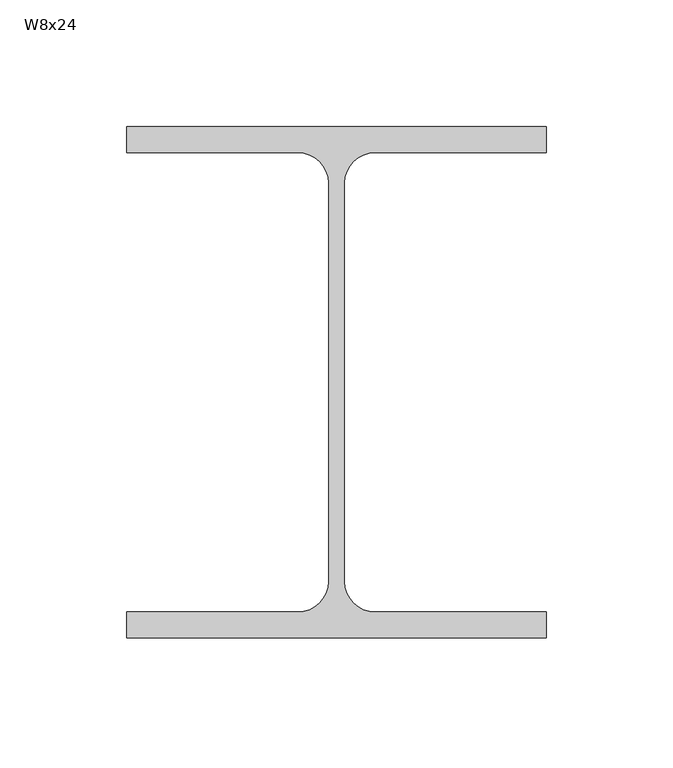
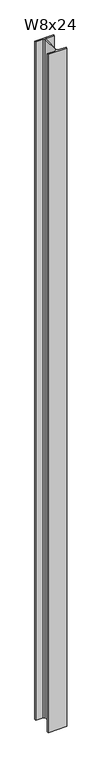
"""IFC4 building model written with IfcOpenShell, lengths in millimetres: column geometry, RME WF - Column : W8x24."""

from ifc_helpers import new_model, si_unit, point, frame, frame_2d, origin, place, context, project, spatial, polyline, circle_curve, trimmed, segment, composite_curve, outline, extrude, source, transform, mapped, element, save


def w8x24_ef2073df(model_context):
    return source(origin(), model_context, "Body", "SweptSolid", [
        extrude(outline(composite_curve([segment(polyline([(82.55, 100.711), (82.55, 90.551), (15.1765, 90.551)]), True, "CONTINUOUS"), segment(trimmed(circle_curve(frame_2d((15.1765, 78.486)), 12.065), [point((15.1765, 90.551))], [point((3.1115, 78.486))], True, "CARTESIAN"), True, "CONTINUOUS"), segment(polyline([(3.1115, 78.486), (3.1115, -78.486)]), True, "CONTINUOUS"), segment(trimmed(circle_curve(frame_2d((15.1765, -78.486)), 12.065), [point((3.1115, -78.486))], [point((15.1765, -90.551))], True, "CARTESIAN"), True, "CONTINUOUS"), segment(polyline([(15.1765, -90.551), (82.55, -90.551), (82.55, -100.711), (-82.55, -100.711), (-82.55, -90.551), (-15.1765, -90.551)]), True, "CONTINUOUS"), segment(trimmed(circle_curve(frame_2d((-15.1765, -78.486)), 12.065), [point((-15.1765, -90.551))], [point((-3.1115, -78.486))], True, "CARTESIAN"), True, "CONTINUOUS"), segment(polyline([(-3.1115, -78.486), (-3.1115, 78.486)]), True, "CONTINUOUS"), segment(trimmed(circle_curve(frame_2d((-15.1765, 78.486)), 12.065), [point((-3.1115, 78.486))], [point((-15.1765, 90.551))], True, "CARTESIAN"), True, "CONTINUOUS"), segment(polyline([(-15.1765, 90.551), (-82.55, 90.551), (-82.55, 100.711), (82.55, 100.711)]), True, "CONTINUOUS")], self_intersect=False)), frame((0.0, 0.0, -304.8), z_axis=(0.0, 0.0, 1.0), x_axis=(1.0, 0.0, 0.0)), (0.0, 0.0, 1.0), 6334.125),
    ])


if __name__ == "__main__":
    model = new_model("IFC4")
    model_context = context("Model", 3, world=origin())
    ifc_project = project(units=[si_unit("LENGTHUNIT", "METRE", prefix="MILLI")], contexts=[model_context])
    site = spatial("IfcSite", under=ifc_project)
    building = spatial("IfcBuilding", under=site)
    placement = place(None, origin())
    w8x24_shape = w8x24_ef2073df(model_context)
    element("IfcColumn", 1, ObjectType="RME WF - Column : W8x24", at=placement, inside=building, context=model_context, shape_type="MappedRepresentation", body=[
        mapped(w8x24_shape, transform((0.0, 0.0, 0.0), x_axis=(1.0, 0.0, 0.0), y_axis=(0.0, 1.0, 0.0), z_axis=(0.0, 0.0, 1.0))),
    ])
    save(model, "model.ifc")

# Revit data of these elements
# Type "RME WF - Column : W8x24"
#   Type Mark = "C1"
#   REINF TYPE [instance default] = ""
#   Nominal Size = "W16"
#   COL REMARKS [instance default] = ""
#   BP [instance default] = ""
#   Assembly Code = "B10"
#   W = 24
#   bf = 0' - 6 1/2"
#   d = 0' - 7.93"
#   k = 0' - 0 7/8"
#   kr = 0' - 0.475"
#   tf = 0' - 0.4"
#   tw = 0' - 0.245"
#   A = 0.0491667 SF
#   Structural Material [instance default] = Metal - Steel - ASTM A992
# Element 1 (IfcColumn, "RME WF - Column : W8x24")
#   Materials on its faces: "Metal - Steel - ASTM A992"
# Materials
#   "Metal - Steel - ASTM A992": class "Metal", colour RGB 255 128 0, transparency 0
